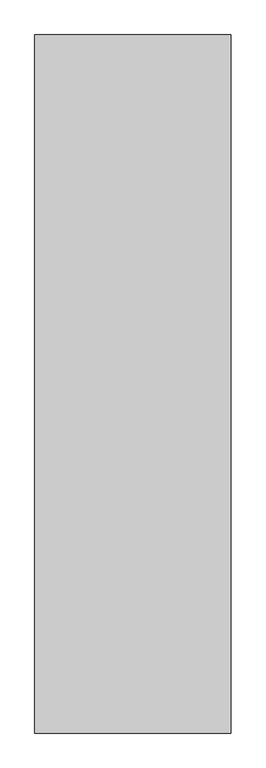
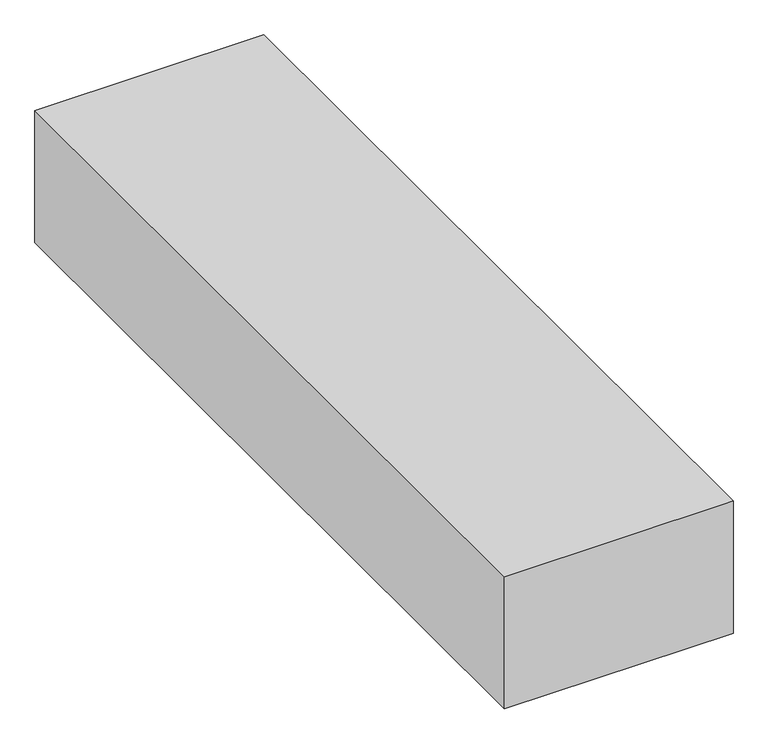
"""IFC4 building model written with IfcOpenShell, lengths in millimetres: proxy geometry, Space Planning Box_hec : Space Planning Box_hec."""

import ifcopenshell
import ifcopenshell.guid

model = None  # the IFC model being written
_history = None  # IfcOwnerHistory: only IFC2X3 demands one
_inside = {}  # id of a spatial element -> (the spatial element, [elements in it])
_under = {}  # id of a project, library or spatial element -> (it, [spatial elements below it])
_declared = {}  # id of a project -> (the project, [libraries it declares])
_typed = {}  # id of a type object -> (the type object, [elements of that type])
_made_of = {}  # id of a material, layer set ... -> (it, [elements and type objects made of it])


def new_model(schema):
    """Start an empty IFC model of exactly this schema.

    Asked for "IFC4X3", IfcOpenShell would pick the latest addendum, in which some entities
    have other attributes; the version numbers below select the first issue.
    IFC2X3 requires an IfcOwnerHistory on every rooted entity: one is made here for all.
    """
    global model, _history
    if schema == "IFC4X3":
        model = ifcopenshell.file(schema_version=(4, 3, 0, 0))
    else:
        model = ifcopenshell.file(schema=schema)
    _inside.clear()
    _under.clear()
    _declared.clear()
    _typed.clear()
    _made_of.clear()
    _history = None
    if model.schema == "IFC2X3":
        org = make("IfcOrganization", Name="unknown")
        user = make(
            "IfcPersonAndOrganization",
            ThePerson=make("IfcPerson", FamilyName="unknown"),
            TheOrganization=org,
        )
        app = make(
            "IfcApplication",
            ApplicationDeveloper=org,
            Version="unknown",
            ApplicationFullName="unknown",
            ApplicationIdentifier="unknown",
        )
        _history = make(
            "IfcOwnerHistory",
            OwningUser=user,
            OwningApplication=app,
            ChangeAction="ADDED",
            CreationDate=0,
        )
    return model


def make(cls, **values):
    """One entity of the class cls with the attributes given. An attribute that is None is left unset."""
    return model.create_entity(
        cls, **{name: value for name, value in values.items() if value is not None}
    )


def rooted(cls, **values):
    """An entity with a GlobalId (a new one), such as an element, a storey or a relation."""
    return make(cls, GlobalId=ifcopenshell.guid.new(), OwnerHistory=_history, **values)


def si_unit(unit_type, name, prefix=None):
    """IfcSIUnit, for example si_unit("LENGTHUNIT", "METRE", prefix="MILLI")."""
    return make("IfcSIUnit", UnitType=unit_type, Prefix=prefix, Name=name)


def assignment(units):
    """IfcUnitAssignment: the units of a project."""
    return None if units is None else make("IfcUnitAssignment", Units=units)


def point(xyz):
    """IfcCartesianPoint."""
    return None if xyz is None else make("IfcCartesianPoint", Coordinates=xyz)


def direction(xyz):
    """IfcDirection."""
    return None if xyz is None else make("IfcDirection", DirectionRatios=xyz)


def frame(location, z_axis=None, x_axis=None):
    """IfcAxis2Placement3D, a coordinate frame: its origin and axes. An axis left out is left unset."""
    return make(
        "IfcAxis2Placement3D",
        Location=point(location),
        Axis=direction(z_axis),
        RefDirection=direction(x_axis),
    )


def origin():
    """The frame at (0, 0, 0) with its axes left unset."""
    return frame((0.0, 0.0, 0.0))


def origin_with_axes():
    """The frame at (0, 0, 0) with the z axis (0, 0, 1) and the x axis (1, 0, 0) written out."""
    return frame((0.0, 0.0, 0.0), z_axis=(0.0, 0.0, 1.0), x_axis=(1.0, 0.0, 0.0))


def place(relative_to, where):
    """IfcLocalPlacement: puts the frame where relative to a parent placement (None: the world)."""
    return make(
        "IfcLocalPlacement", PlacementRelTo=relative_to, RelativePlacement=where
    )


def context(
    kind, dimensions, precision=None, world=None, true_north=None, identifier=None
):
    """IfcGeometricRepresentationContext, for example the 3D "Model" context."""
    return make(
        "IfcGeometricRepresentationContext",
        ContextIdentifier=identifier,
        ContextType=kind,
        CoordinateSpaceDimension=dimensions,
        Precision=precision,
        WorldCoordinateSystem=world,
        TrueNorth=true_north,
    )


def project(units=None, contexts=None):
    """IfcProject with its units and contexts."""
    return rooted(
        "IfcProject",
        Name="project",
        RepresentationContexts=contexts,
        UnitsInContext=assignment(units),
    )


def spatial(cls, under=None, at=None, **own):
    """A site, building, storey or space (cls), placed at a placement, below another one or the project."""
    s = rooted(cls, ObjectPlacement=at, **own)
    if under is not None:
        _under.setdefault(under.id(), (under, []))[1].append(s)
    return s


def polyline(points):
    """IfcPolyline through the points."""
    return make("IfcPolyline", Points=[point(p) for p in points])


def outline(outer, holes=None, kind="AREA"):
    """IfcArbitraryClosedProfileDef: a profile drawn as a closed curve; with holes, ...WithVoids."""
    if holes is None:
        return make("IfcArbitraryClosedProfileDef", ProfileType=kind, OuterCurve=outer)
    return make(
        "IfcArbitraryProfileDefWithVoids",
        ProfileType=kind,
        OuterCurve=outer,
        InnerCurves=holes,
    )


def extrude(swept, where, along, depth):
    """IfcExtrudedAreaSolid: the profile swept, set in the frame where, extruded along a direction by depth."""
    return make(
        "IfcExtrudedAreaSolid",
        SweptArea=swept,
        Position=where,
        ExtrudedDirection=direction(along),
        Depth=depth,
    )


def shape(context_of_items, identifier, shape_type, items):
    """IfcShapeRepresentation: the items that make up one representation, for example the "Body"."""
    return make(
        "IfcShapeRepresentation",
        ContextOfItems=context_of_items,
        RepresentationIdentifier=identifier,
        RepresentationType=shape_type,
        Items=items,
    )


def source(mapping_origin, context_of_items, identifier, shape_type, items):
    """IfcRepresentationMap: a shape defined once, which mapped items show again and again."""
    return make(
        "IfcRepresentationMap",
        MappingOrigin=mapping_origin,
        MappedRepresentation=shape(context_of_items, identifier, shape_type, items),
    )


def transform(
    local_origin,
    x_axis=None,
    y_axis=None,
    z_axis=None,
    scale=None,
    scale2=None,
    scale3=None,
    uniform=True,
):
    """IfcCartesianTransformationOperator3D, or its non-uniform kind. x_axis, y_axis, z_axis: its Axis1, 2, 3."""
    if uniform:
        return make(
            "IfcCartesianTransformationOperator3D",
            Axis1=direction(x_axis),
            Axis2=direction(y_axis),
            LocalOrigin=point(local_origin),
            Scale=scale,
            Axis3=direction(z_axis),
        )
    return make(
        "IfcCartesianTransformationOperator3DnonUniform",
        Axis1=direction(x_axis),
        Axis2=direction(y_axis),
        LocalOrigin=point(local_origin),
        Scale=scale,
        Axis3=direction(z_axis),
        Scale2=scale2,
        Scale3=scale3,
    )


def mapped(mapping_source, mapping_target):
    """IfcMappedItem: shows the shape of a source again, moved by a transform."""
    return make(
        "IfcMappedItem", MappingSource=mapping_source, MappingTarget=mapping_target
    )


def made_of(thing, what):
    """Note that an element or type object is made of a material, layer set ...; save() writes the relation."""
    if what is not None:
        _made_of.setdefault(what.id(), (what, []))[1].append(thing)
    return thing


def element(
    cls,
    number,
    at=None,
    inside=None,
    cuts=None,
    type_object=None,
    material=None,
    context=None,
    identifier="Body",
    shape_type=None,
    held_by="IfcProductDefinitionShape",
    body=None,
    shapes=None,
    **own,
):
    """One element of the class cls, such as IfcWall. Its Tag is "e" and its number.

    at: its placement. inside: the storey or other place that contains it. cuts: it is an
    opening in that element (IfcRelVoidsElement). A single representation is given by context,
    identifier, shape_type and body (its items); several are given by shapes. held_by: the class
    of the entity that holds the representations. save() writes the other relations.
    """
    e = rooted(cls, Tag="e%d" % number, ObjectPlacement=at, **own)
    if body is not None:
        shapes = [shape(context, identifier, shape_type, body)]
    if shapes is not None:
        e.Representation = make(held_by, Representations=shapes)
    if inside is not None:
        _inside.setdefault(inside.id(), (inside, []))[1].append(e)
    if cuts is not None:
        rooted(
            "IfcRelVoidsElement", RelatingBuildingElement=cuts, RelatedOpeningElement=e
        )
    if type_object is not None:
        _typed.setdefault(type_object.id(), (type_object, []))[1].append(e)
    return made_of(e, material)


def aggregate(whole, parts):
    """IfcRelAggregates: a whole, such as a stair, and the parts it consists of."""
    return rooted("IfcRelAggregates", RelatingObject=whole, RelatedObjects=parts)


def save(model, path):
    """Write the relations noted so far, then the file.

    IfcRelAggregates (storeys below a building ...), IfcRelContainedInSpatialStructure (elements
    in a storey), IfcRelDefinesByType, IfcRelAssociatesMaterial and IfcRelDeclares: one each for
    every whole, place, type object, material and project.
    """
    for whole, parts in _under.values():
        aggregate(whole, parts)
    for where, things in _inside.values():
        rooted(
            "IfcRelContainedInSpatialStructure",
            RelatedElements=things,
            RelatingStructure=where,
        )
    for kind, things in _typed.values():
        rooted("IfcRelDefinesByType", RelatedObjects=things, RelatingType=kind)
    for what, things in _made_of.values():
        rooted("IfcRelAssociatesMaterial", RelatedObjects=things, RelatingMaterial=what)
    for by, libraries in _declared.values():
        rooted("IfcRelDeclares", RelatingContext=by, RelatedDefinitions=libraries)
    model.write(path)


def generic_models_50f5a469(model_context):
    return source(origin(), model_context, "Body", "SweptSolid", [
        extrude(outline(polyline([(4500.0, 16000.0), (4500.0, -16000.0), (-4500.0, -16000.0), (-4500.0, 16000.0), (4500.0, 16000.0)])), origin_with_axes(), (0.0, 0.0, 1.0), 5500.0),
    ])


if __name__ == "__main__":
    model = new_model("IFC4")
    model_context = context("Model", 3, world=origin())
    ifc_project = project(units=[si_unit("LENGTHUNIT", "METRE", prefix="MILLI")], contexts=[model_context])
    site = spatial("IfcSite", under=ifc_project)
    building = spatial("IfcBuilding", under=site)
    placement = place(None, origin())
    generic_models_shape = generic_models_50f5a469(model_context)
    element("IfcBuildingElementProxy", 1, Name="Space Planning Box_hec : Space Planning Box_hec", ObjectType="Space Planning Box_hec : Space Planning Box_hec", at=placement, inside=building, context=model_context, shape_type="MappedRepresentation", body=[
        mapped(generic_models_shape, transform((0.0, 0.0, 0.0), x_axis=(1.0, 0.0, 0.0), y_axis=(0.0, 1.0, 0.0), z_axis=(0.0, 0.0, 1.0))),
    ])
    save(model, "model.ifc")

# Revit data of these elements
# Type "Space Planning Box_hec : Space Planning Box_hec"
#   Type Comments = "..."
#   Room Name [instance default] = "?"
#   Interior Finish [instance default] = ""
#   Exterior Finish [instance default] = ""
#   Department [instance default] = ""
#   Assembly Code = "..."
#   ceiling height [instance default] = 0
#   Width [instance default] = 1524 mm
#   Program Area [instance default] = 0.00 m²
#   Length [instance default] = 1524 mm
#   Height [instance default] = 1524 mm
#   Area [instance default] = 2.32258 m²
#   Fill Color [instance default] = Cyan
#   Default Elevation = 0
# Element 1 (IfcBuildingElementProxy, "Space Planning Box_hec : Space Planning Box_hec")
#   Room Name = "Electrical Room-1"
#   Exterior Finish = "N/A..N/A,,EW1..EW2..N/A"
#   Department = "CI"
#   Width = 9000 mm
#   Program Area = 306.00 m²
#   Length = 32000 mm
#   Height = 5500 mm
#   Area = 288.00 m²
#   Fill Color = Yellow
#   Materials on its faces: "Yellow"
# Materials
#   "Cyan": class "Generic", colour RGB 0 255 255, transparency 0.2, Cost = 0
#   "Yellow": class "Generic", colour RGB 255 255 0, transparency 0.2, Cost = 0
